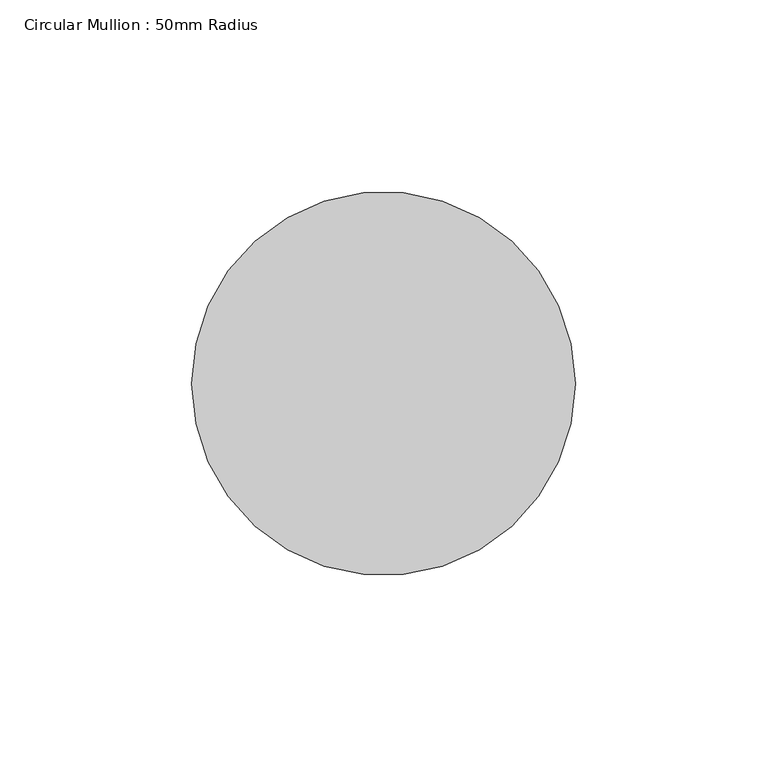
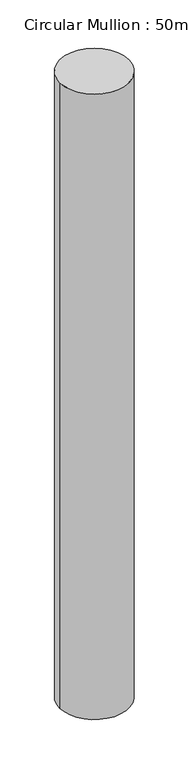
"""IFC4 building model written with IfcOpenShell, lengths in millimetres: member geometry, Circular Mullion : 50mm Radius."""

from ifc_helpers import new_model, si_unit, point, frame, origin, origin_2d, place, context, project, spatial, circle_curve, trimmed, segment, composite_curve, outline, extrude, source, transform, mapped, element, save


def circular_mullion_50mm_radius_2f31d31a(model_context):
    return source(origin(), model_context, "Body", "SweptSolid", [
        extrude(outline(composite_curve([segment(trimmed(circle_curve(origin_2d(), 50.0), [point((50.0, 0.0))], [point((-50.0, 0.0))], False, "CARTESIAN"), True, "CONTINUOUS"), segment(trimmed(circle_curve(origin_2d(), 50.0), [point((-50.0, 0.0))], [point((50.0, 0.0))], False, "CARTESIAN"), True, "CONTINUOUS")], self_intersect=False)), frame((0.0, 0.0, -955.3724204), z_axis=(0.0, 0.0, 1.0), x_axis=(1.0, 0.0, 0.0)), (0.0, 0.0, 1.0), 955.3724204),
    ])


if __name__ == "__main__":
    model = new_model("IFC4")
    model_context = context("Model", 3, world=origin())
    ifc_project = project(units=[si_unit("LENGTHUNIT", "METRE", prefix="MILLI")], contexts=[model_context])
    site = spatial("IfcSite", under=ifc_project)
    building = spatial("IfcBuilding", under=site)
    placement = place(None, origin())
    circular_mullion_50mm_radius_shape = circular_mullion_50mm_radius_2f31d31a(model_context)
    element("IfcMember", 1, ObjectType="Circular Mullion : 50mm Radius", at=placement, inside=building, context=model_context, shape_type="MappedRepresentation", body=[
        mapped(circular_mullion_50mm_radius_shape, transform((0.0, 0.0, 0.0), x_axis=(1.0, 0.0, 0.0), y_axis=(0.0, 1.0, 0.0), z_axis=(0.0, 0.0, 1.0))),
    ])
    save(model, "model.ifc")

# Revit data of these elements
# Type "Circular Mullion : 50mm Radius"
#   built-in parameter 1007350 = 0.164042 (stored number, unit not read)
# Element 1 (IfcMember, "Circular Mullion : 50mm Radius")
#   Materials on its faces: "Aluminium"
# Materials
#   "Aluminium": class "Metal", colour RGB 247 247 247, transparency 0, Description = "Aluminium 6061", Cost = 0
